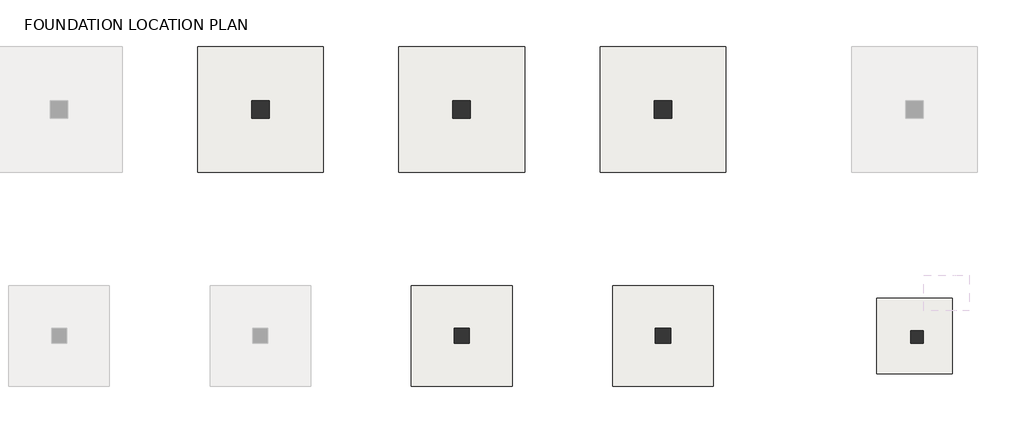
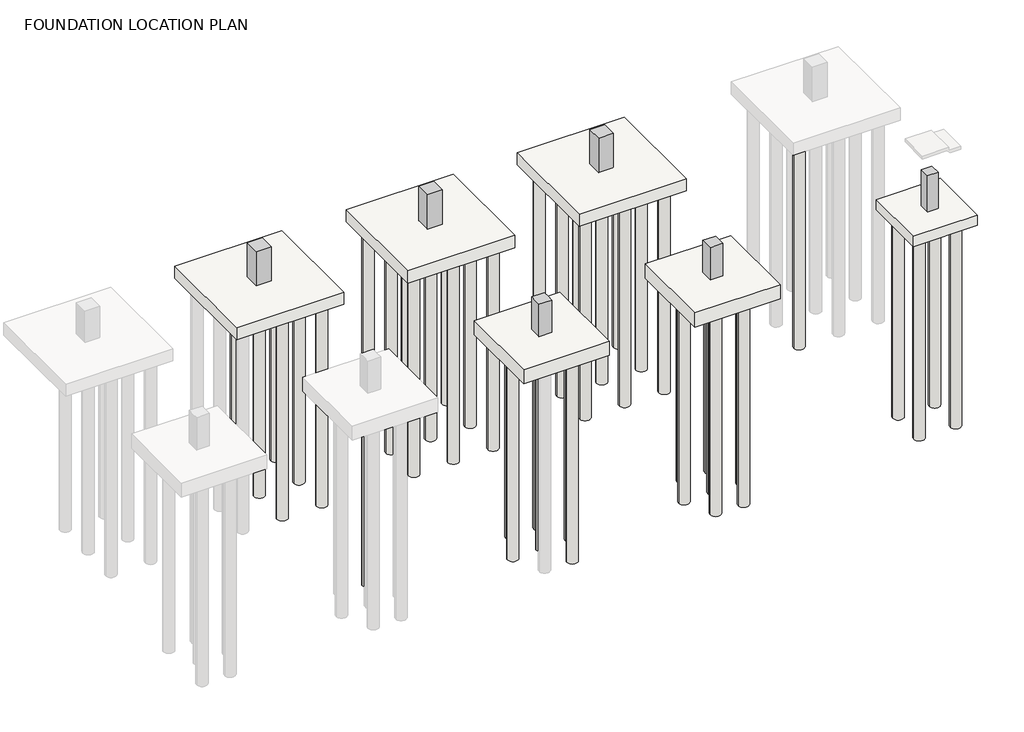
# One storey, part 2 of 3: 49 slabs, 6 columns.
"""IFC4 building model written with IfcOpenShell, lengths in millimetres."""

from ifc_helpers import new_model, si_unit, point, frame, frame_2d, origin, place, context, project, spatial, polyline, circle_curve, trimmed, segment, composite_curve, outline, extrude, faceted_brep, element, save

model = new_model("IFC4")

# Units and contexts
model_context = context("Model", 3, world=origin())
ifc_project = project(units=[si_unit("LENGTHUNIT", "METRE", prefix="MILLI")], contexts=[model_context])

# Site, building, storey
site = spatial("IfcSite", under=ifc_project)
building = spatial("IfcBuilding", under=site)
storey = spatial("IfcBuildingStorey", under=building, Name="FOUNDATION LOCATION PLAN", Elevation=-1699.994759)

# Columns
placement = place(None, origin())
element("IfcColumn", 1, ObjectType="Concrete-Rectangular-Column_R1 : CLS111_RC COLUMN_UG_C1", at=placement, inside=storey, context=model_context, shape_type="Brep", body=[
    faceted_brep([(41850.0, 21199.5208589, -1199.994759), (42350.0, 21199.5208589, -1199.994759), (42350.0, 20699.5208589, -1199.994759), (41850.0, 20699.5208589, -1199.994759), (41850.0, 21199.5208589, 450.005241), (41850.0, 21199.5208589, 600.005241), (42000.0, 21199.5208589, 600.005241), (42350.0, 21199.5208589, 600.005241), (41850.0, 20699.5208589, 600.005241), (41850.0, 20999.5208589, 600.005241), (42350.0, 20699.5208589, 600.005241)], [[[0, 1, 2, 3]], [[1, 0, 4, 5, 6, 7]], [[0, 3, 8, 9, 5, 4]], [[3, 2, 10, 8]], [[2, 1, 7, 10]], [[8, 10, 7, 6, 5, 9]]]),
])
element("IfcColumn", 2, ObjectType="Concrete-Rectangular-Column_R1 : CLS111_RC COLUMN_UG_C3", at=placement, inside=storey, context=model_context, shape_type="Brep", body=[
    faceted_brep([(15650.0, 30349.5208589, -1099.994759), (16350.0, 30349.5208589, -1099.994759), (16350.0, 29649.5208589, -1099.994759), (15650.0, 29649.5208589, -1099.994759), (15650.0, 30349.5208589, 450.005241), (15650.0, 30349.5208589, 600.005241), (16350.0, 30349.5208589, 600.005241), (16350.0, 30349.5208589, 450.005241), (16350.0, 29649.5208589, 600.005241), (16350.0, 29649.5208589, 450.005241), (15650.0, 29649.5208589, 600.005241), (15650.0, 29649.5208589, 450.005241)], [[[0, 1, 2, 3]], [[1, 0, 4, 5, 6, 7]], [[2, 1, 7, 6, 8, 9]], [[3, 2, 9, 8, 10, 11]], [[0, 3, 11, 10, 5, 4]], [[6, 5, 10, 8]]]),
])
element("IfcColumn", 3, ObjectType="Concrete-Rectangular-Column_R1 : CLS111_RC COLUMN_UG_C3", at=placement, inside=storey, context=model_context, shape_type="Brep", body=[
    faceted_brep([(23650.0, 30349.5208589, -1099.994759), (24350.0, 30349.5208589, -1099.994759), (24350.0, 29649.5208589, -1099.994759), (23650.0, 29649.5208589, -1099.994759), (23650.0, 30349.5208589, 450.005241), (23650.0, 30349.5208589, 600.005241), (24350.0, 30349.5208589, 600.005241), (24350.0, 30349.5208589, 450.005241), (24350.0, 29649.5208589, 600.005241), (24350.0, 29649.5208589, 450.005241), (23650.0, 29649.5208589, 600.005241), (23650.0, 29649.5208589, 450.005241)], [[[0, 1, 2, 3]], [[1, 0, 4, 5, 6, 7]], [[2, 1, 7, 6, 8, 9]], [[3, 2, 9, 8, 10, 11]], [[0, 3, 11, 10, 5, 4]], [[6, 5, 10, 8]]]),
])
element("IfcColumn", 4, ObjectType="Concrete-Rectangular-Column_R1 : CLS111_RC COLUMN_UG_C3", at=placement, inside=storey, context=model_context, shape_type="Brep", body=[
    faceted_brep([(31650.0, 30349.5208589, -1099.994759), (32350.0, 30349.5208589, -1099.994759), (32350.0, 29649.5208589, -1099.994759), (31650.0, 29649.5208589, -1099.994759), (31650.0, 30349.5208589, 450.005241), (31650.0, 30349.5208589, 600.005241), (32350.0, 30349.5208589, 600.005241), (32350.0, 30349.5208589, 450.005241), (32350.0, 29649.5208589, 600.005241), (32350.0, 29649.5208589, 450.005241), (31650.0, 29649.5208589, 600.005241), (31650.0, 29649.5208589, 450.005241)], [[[0, 1, 2, 3]], [[1, 0, 4, 5, 6, 7]], [[2, 1, 7, 6, 8, 9]], [[3, 2, 9, 8, 10, 11]], [[0, 3, 11, 10, 5, 4]], [[6, 5, 10, 8]]]),
])
element("IfcColumn", 5, ObjectType="Concrete-Rectangular-Column_R1 : CLS111_RC COLUMN_UG_C2", at=placement, inside=storey, context=model_context, shape_type="Brep", body=[
    faceted_brep([(23700.0, 21299.5208589, -999.994759), (24300.0, 21299.5208589, -999.994759), (24300.0, 20699.5208589, -999.994759), (23700.0, 20699.5208589, -999.994759), (23700.0, 21299.5208589, 450.005241), (23700.0, 21299.5208589, 600.005241), (24300.0, 21299.5208589, 600.005241), (24300.0, 21299.5208589, 450.005241), (24300.0, 20999.5208589, 600.005241), (24300.0, 20699.5208589, 600.005241), (23700.0, 20699.5208589, 600.005241), (23700.0, 20999.5208589, 600.005241)], [[[0, 1, 2, 3]], [[1, 0, 4, 5, 6, 7]], [[2, 1, 7, 6, 8, 9]], [[3, 2, 9, 10]], [[0, 3, 10, 11, 5, 4]], [[6, 5, 11, 10, 9, 8]]]),
])
element("IfcColumn", 6, ObjectType="Concrete-Rectangular-Column_R1 : CLS111_RC COLUMN_UG_C2", at=placement, inside=storey, context=model_context, shape_type="Brep", body=[
    faceted_brep([(31700.0, 21299.5208589, -999.994759), (32300.0, 21299.5208589, -999.994759), (32300.0, 20699.5208589, -999.994759), (31700.0, 20699.5208589, -999.994759), (31700.0, 21299.5208589, 450.005241), (31700.0, 21299.5208589, 600.005241), (32300.0, 21299.5208589, 600.005241), (32300.0, 21299.5208589, 450.005241), (32300.0, 20999.5208589, 600.005241), (32300.0, 20699.5208589, 600.005241), (31700.0, 20699.5208589, 600.005241), (31700.0, 20999.5208589, 600.005241)], [[[0, 1, 2, 3]], [[1, 0, 4, 5, 6, 7]], [[2, 1, 7, 6, 8, 9]], [[3, 2, 9, 10]], [[0, 3, 10, 11, 5, 4]], [[6, 5, 11, 10, 9, 8]]]),
])

# Slabs
element("IfcSlab", 7, ObjectType="Footing-Rectangular_R1 : FTS301_Footing-Rectangular_3000x3000x500_F1", at=placement, inside=storey, context=model_context, shape_type="SweptSolid", body=[
    extrude(outline(polyline([(43500.0, 22499.5208589), (43500.0, 19499.5208589), (40500.0, 19499.5208589), (40500.0, 22499.5208589), (43500.0, 22499.5208589)])), frame((0.0, 0.0, -1699.994759), z_axis=(0.0, 0.0, 1.0), x_axis=(1.0, 0.0, 0.0)), (0.0, 0.0, 1.0), 500.0),
])
element("IfcSlab", 8, ObjectType="Footing-Rectangular_R1 : FTS301_Footing-Rectangular_4000x4000x700_F2", at=placement, inside=storey, context=model_context, shape_type="SweptSolid", body=[
    extrude(outline(polyline([(26000.0, 22999.5208589), (26000.0, 18999.5208589), (22000.0, 18999.5208589), (22000.0, 22999.5208589), (26000.0, 22999.5208589)])), frame((0.0, 0.0, -1699.994759), z_axis=(0.0, 0.0, 1.0), x_axis=(1.0, 0.0, 0.0)), (0.0, 0.0, 1.0), 700.0),
])
element("IfcSlab", 9, ObjectType="Footing-Rectangular_R1 : FTS301_Footing-Rectangular_4000x4000x700_F2", at=placement, inside=storey, context=model_context, shape_type="SweptSolid", body=[
    extrude(outline(polyline([(34000.0, 22999.5208589), (34000.0, 18999.5208589), (30000.0, 18999.5208589), (30000.0, 22999.5208589), (34000.0, 22999.5208589)])), frame((0.0, 0.0, -1699.994759), z_axis=(0.0, 0.0, 1.0), x_axis=(1.0, 0.0, 0.0)), (0.0, 0.0, 1.0), 700.0),
])
element("IfcSlab", 10, ObjectType="Footing-Rectangular_R1 : FTS301_Footing-Rectangular_5000x5000x600_F3", at=placement, inside=storey, context=model_context, shape_type="SweptSolid", body=[
    extrude(outline(polyline([(18500.0, 32499.5208589), (18500.0, 27499.5208589), (13500.0, 27499.5208589), (13500.0, 32499.5208589), (18500.0, 32499.5208589)])), frame((0.0, 0.0, -1699.994759), z_axis=(0.0, 0.0, 1.0), x_axis=(1.0, 0.0, 0.0)), (0.0, 0.0, 1.0), 600.0),
])
element("IfcSlab", 11, ObjectType="Footing-Rectangular_R1 : FTS301_Footing-Rectangular_5000x5000x600_F3", at=placement, inside=storey, context=model_context, shape_type="SweptSolid", body=[
    extrude(outline(polyline([(26500.0, 32499.5208589), (26500.0, 27499.5208589), (21500.0, 27499.5208589), (21500.0, 32499.5208589), (26500.0, 32499.5208589)])), frame((0.0, 0.0, -1699.994759), z_axis=(0.0, 0.0, 1.0), x_axis=(1.0, 0.0, 0.0)), (0.0, 0.0, 1.0), 600.0),
])
element("IfcSlab", 12, ObjectType="Footing-Rectangular_R1 : FTS301_Footing-Rectangular_5000x5000x600_F3", at=placement, inside=storey, context=model_context, shape_type="SweptSolid", body=[
    extrude(outline(polyline([(34500.0, 32499.5208589), (34500.0, 27499.5208589), (29500.0, 27499.5208589), (29500.0, 32499.5208589), (34500.0, 32499.5208589)])), frame((0.0, 0.0, -1699.994759), z_axis=(0.0, 0.0, 1.0), x_axis=(1.0, 0.0, 0.0)), (0.0, 0.0, 1.0), 600.0),
])
element("IfcSlab", 13, ObjectType="HEC_PILE : FTPS102_D500", at=placement, inside=storey, context=model_context, shape_type="SweptSolid", body=[
    extrude(outline(composite_curve([segment(trimmed(circle_curve(frame_2d((41150.0, 21849.5208589)), 250.0), [point((41400.0, 21849.5208589))], [point((40900.0, 21849.5208589))], False, "CARTESIAN"), True, "CONTINUOUS"), segment(trimmed(circle_curve(frame_2d((41150.0, 21849.5208589)), 250.0), [point((40900.0, 21849.5208589))], [point((41400.0, 21849.5208589))], False, "CARTESIAN"), True, "CONTINUOUS")], self_intersect=False)), frame((0.0, 0.0, -11749.994759), z_axis=(0.0, 0.0, 1.0), x_axis=(1.0, 0.0, 0.0)), (0.0, 0.0, 1.0), 10150.0),
])
element("IfcSlab", 14, ObjectType="HEC_PILE : FTPS102_D500", at=placement, inside=storey, context=model_context, shape_type="SweptSolid", body=[
    extrude(outline(composite_curve([segment(trimmed(circle_curve(frame_2d((42850.0, 21849.5208589)), 250.0), [point((42600.0, 21849.5208589))], [point((43100.0, 21849.5208589))], False, "CARTESIAN"), True, "CONTINUOUS"), segment(trimmed(circle_curve(frame_2d((42850.0, 21849.5208589)), 250.0), [point((43100.0, 21849.5208589))], [point((42600.0, 21849.5208589))], False, "CARTESIAN"), True, "CONTINUOUS")], self_intersect=False)), frame((0.0, 0.0, -11749.994759), z_axis=(0.0, 0.0, 1.0), x_axis=(1.0, 0.0, 0.0)), (0.0, 0.0, 1.0), 10150.0),
])
element("IfcSlab", 15, ObjectType="HEC_PILE : FTPS102_D500", at=placement, inside=storey, context=model_context, shape_type="SweptSolid", body=[
    extrude(outline(composite_curve([segment(trimmed(circle_curve(frame_2d((41150.0, 20149.5208589)), 250.0), [point((41400.0, 20149.5208589))], [point((40900.0, 20149.5208589))], False, "CARTESIAN"), True, "CONTINUOUS"), segment(trimmed(circle_curve(frame_2d((41150.0, 20149.5208589)), 250.0), [point((40900.0, 20149.5208589))], [point((41400.0, 20149.5208589))], False, "CARTESIAN"), True, "CONTINUOUS")], self_intersect=False)), frame((0.0, 0.0, -11749.994759), z_axis=(0.0, 0.0, 1.0), x_axis=(1.0, 0.0, 0.0)), (0.0, 0.0, 1.0), 10150.0),
])
element("IfcSlab", 16, ObjectType="HEC_PILE : FTPS102_D500", at=placement, inside=storey, context=model_context, shape_type="SweptSolid", body=[
    extrude(outline(composite_curve([segment(trimmed(circle_curve(frame_2d((42850.0, 20149.5208589)), 250.0), [point((42600.0, 20149.5208589))], [point((43100.0, 20149.5208589))], False, "CARTESIAN"), True, "CONTINUOUS"), segment(trimmed(circle_curve(frame_2d((42850.0, 20149.5208589)), 250.0), [point((43100.0, 20149.5208589))], [point((42600.0, 20149.5208589))], False, "CARTESIAN"), True, "CONTINUOUS")], self_intersect=False)), frame((0.0, 0.0, -11749.994759), z_axis=(0.0, 0.0, 1.0), x_axis=(1.0, 0.0, 0.0)), (0.0, 0.0, 1.0), 10150.0),
])
element("IfcSlab", 17, ObjectType="HEC_PILE : FTPS102_D500", at=placement, inside=storey, context=model_context, shape_type="SweptSolid", body=[
    extrude(outline(composite_curve([segment(trimmed(circle_curve(frame_2d((16650.0, 22349.5208589)), 250.0), [point((16400.0, 22349.5208589))], [point((16900.0, 22349.5208589))], False, "CARTESIAN"), True, "CONTINUOUS"), segment(trimmed(circle_curve(frame_2d((16650.0, 22349.5208589)), 250.0), [point((16900.0, 22349.5208589))], [point((16400.0, 22349.5208589))], False, "CARTESIAN"), True, "CONTINUOUS")], self_intersect=False)), frame((0.0, 0.0, -11749.994759), z_axis=(0.0, 0.0, 1.0), x_axis=(1.0, 0.0, 0.0)), (0.0, 0.0, 1.0), 10150.0),
])
element("IfcSlab", 18, ObjectType="HEC_PILE : FTPS102_D500", at=placement, inside=storey, context=model_context, shape_type="SweptSolid", body=[
    extrude(outline(composite_curve([segment(trimmed(circle_curve(frame_2d((24650.0, 19649.5208589)), 250.0), [point((24400.0, 19649.5208589))], [point((24900.0, 19649.5208589))], False, "CARTESIAN"), True, "CONTINUOUS"), segment(trimmed(circle_curve(frame_2d((24650.0, 19649.5208589)), 250.0), [point((24900.0, 19649.5208589))], [point((24400.0, 19649.5208589))], False, "CARTESIAN"), True, "CONTINUOUS")], self_intersect=False)), frame((0.0, 0.0, -11749.994759), z_axis=(0.0, 0.0, 1.0), x_axis=(1.0, 0.0, 0.0)), (0.0, 0.0, 1.0), 10150.0),
])
element("IfcSlab", 19, ObjectType="HEC_PILE : FTPS102_D500", at=placement, inside=storey, context=model_context, shape_type="SweptSolid", body=[
    extrude(outline(composite_curve([segment(trimmed(circle_curve(frame_2d((22650.0, 20999.5208589)), 250.0), [point((22900.0, 20999.5208589))], [point((22400.0, 20999.5208589))], False, "CARTESIAN"), True, "CONTINUOUS"), segment(trimmed(circle_curve(frame_2d((22650.0, 20999.5208589)), 250.0), [point((22400.0, 20999.5208589))], [point((22900.0, 20999.5208589))], False, "CARTESIAN"), True, "CONTINUOUS")], self_intersect=False)), frame((0.0, 0.0, -11749.994759), z_axis=(0.0, 0.0, 1.0), x_axis=(1.0, 0.0, 0.0)), (0.0, 0.0, 1.0), 10150.0),
])
element("IfcSlab", 20, ObjectType="HEC_PILE : FTPS102_D500", at=placement, inside=storey, context=model_context, shape_type="SweptSolid", body=[
    extrude(outline(composite_curve([segment(trimmed(circle_curve(frame_2d((24000.0, 20999.5208589)), 250.0), [point((24250.0, 20999.5208589))], [point((23750.0, 20999.5208589))], False, "CARTESIAN"), True, "CONTINUOUS"), segment(trimmed(circle_curve(frame_2d((24000.0, 20999.5208589)), 250.0), [point((23750.0, 20999.5208589))], [point((24250.0, 20999.5208589))], False, "CARTESIAN"), True, "CONTINUOUS")], self_intersect=False)), frame((0.0, 0.0, -11749.994759), z_axis=(0.0, 0.0, 1.0), x_axis=(1.0, 0.0, 0.0)), (0.0, 0.0, 1.0), 10150.0),
])
element("IfcSlab", 21, ObjectType="HEC_PILE : FTPS102_D500", at=placement, inside=storey, context=model_context, shape_type="SweptSolid", body=[
    extrude(outline(composite_curve([segment(trimmed(circle_curve(frame_2d((25350.0, 20999.5208589)), 250.0), [point((25100.0, 20999.5208589))], [point((25600.0, 20999.5208589))], False, "CARTESIAN"), True, "CONTINUOUS"), segment(trimmed(circle_curve(frame_2d((25350.0, 20999.5208589)), 250.0), [point((25600.0, 20999.5208589))], [point((25100.0, 20999.5208589))], False, "CARTESIAN"), True, "CONTINUOUS")], self_intersect=False)), frame((0.0, 0.0, -11749.994759), z_axis=(0.0, 0.0, 1.0), x_axis=(1.0, 0.0, 0.0)), (0.0, 0.0, 1.0), 10150.0),
])
element("IfcSlab", 22, ObjectType="HEC_PILE : FTPS102_D500", at=placement, inside=storey, context=model_context, shape_type="SweptSolid", body=[
    extrude(outline(composite_curve([segment(trimmed(circle_curve(frame_2d((23350.0, 22349.5208589)), 250.0), [point((23600.0, 22349.5208589))], [point((23100.0, 22349.5208589))], False, "CARTESIAN"), True, "CONTINUOUS"), segment(trimmed(circle_curve(frame_2d((23350.0, 22349.5208589)), 250.0), [point((23100.0, 22349.5208589))], [point((23600.0, 22349.5208589))], False, "CARTESIAN"), True, "CONTINUOUS")], self_intersect=False)), frame((0.0, 0.0, -11749.994759), z_axis=(0.0, 0.0, 1.0), x_axis=(1.0, 0.0, 0.0)), (0.0, 0.0, 1.0), 10150.0),
])
element("IfcSlab", 23, ObjectType="HEC_PILE : FTPS102_D500", at=placement, inside=storey, context=model_context, shape_type="SweptSolid", body=[
    extrude(outline(composite_curve([segment(trimmed(circle_curve(frame_2d((24650.0, 22349.5208589)), 250.0), [point((24400.0, 22349.5208589))], [point((24900.0, 22349.5208589))], False, "CARTESIAN"), True, "CONTINUOUS"), segment(trimmed(circle_curve(frame_2d((24650.0, 22349.5208589)), 250.0), [point((24900.0, 22349.5208589))], [point((24400.0, 22349.5208589))], False, "CARTESIAN"), True, "CONTINUOUS")], self_intersect=False)), frame((0.0, 0.0, -11749.994759), z_axis=(0.0, 0.0, 1.0), x_axis=(1.0, 0.0, 0.0)), (0.0, 0.0, 1.0), 10150.0),
])
element("IfcSlab", 24, ObjectType="HEC_PILE : FTPS102_D500", at=placement, inside=storey, context=model_context, shape_type="SweptSolid", body=[
    extrude(outline(composite_curve([segment(trimmed(circle_curve(frame_2d((31350.0, 19649.5208589)), 250.0), [point((31600.0, 19649.5208589))], [point((31100.0, 19649.5208589))], False, "CARTESIAN"), True, "CONTINUOUS"), segment(trimmed(circle_curve(frame_2d((31350.0, 19649.5208589)), 250.0), [point((31100.0, 19649.5208589))], [point((31600.0, 19649.5208589))], False, "CARTESIAN"), True, "CONTINUOUS")], self_intersect=False)), frame((0.0, 0.0, -11749.994759), z_axis=(0.0, 0.0, 1.0), x_axis=(1.0, 0.0, 0.0)), (0.0, 0.0, 1.0), 10150.0),
])
element("IfcSlab", 25, ObjectType="HEC_PILE : FTPS102_D500", at=placement, inside=storey, context=model_context, shape_type="SweptSolid", body=[
    extrude(outline(composite_curve([segment(trimmed(circle_curve(frame_2d((32650.0, 19649.5208589)), 250.0), [point((32400.0, 19649.5208589))], [point((32900.0, 19649.5208589))], False, "CARTESIAN"), True, "CONTINUOUS"), segment(trimmed(circle_curve(frame_2d((32650.0, 19649.5208589)), 250.0), [point((32900.0, 19649.5208589))], [point((32400.0, 19649.5208589))], False, "CARTESIAN"), True, "CONTINUOUS")], self_intersect=False)), frame((0.0, 0.0, -11749.994759), z_axis=(0.0, 0.0, 1.0), x_axis=(1.0, 0.0, 0.0)), (0.0, 0.0, 1.0), 10150.0),
])
element("IfcSlab", 26, ObjectType="HEC_PILE : FTPS102_D500", at=placement, inside=storey, context=model_context, shape_type="SweptSolid", body=[
    extrude(outline(composite_curve([segment(trimmed(circle_curve(frame_2d((30650.0, 20999.5208589)), 250.0), [point((30900.0, 20999.5208589))], [point((30400.0, 20999.5208589))], False, "CARTESIAN"), True, "CONTINUOUS"), segment(trimmed(circle_curve(frame_2d((30650.0, 20999.5208589)), 250.0), [point((30400.0, 20999.5208589))], [point((30900.0, 20999.5208589))], False, "CARTESIAN"), True, "CONTINUOUS")], self_intersect=False)), frame((0.0, 0.0, -11749.994759), z_axis=(0.0, 0.0, 1.0), x_axis=(1.0, 0.0, 0.0)), (0.0, 0.0, 1.0), 10150.0),
])
element("IfcSlab", 27, ObjectType="HEC_PILE : FTPS102_D500", at=placement, inside=storey, context=model_context, shape_type="SweptSolid", body=[
    extrude(outline(composite_curve([segment(trimmed(circle_curve(frame_2d((32000.0, 20999.5208589)), 250.0), [point((32250.0, 20999.5208589))], [point((31750.0, 20999.5208589))], False, "CARTESIAN"), True, "CONTINUOUS"), segment(trimmed(circle_curve(frame_2d((32000.0, 20999.5208589)), 250.0), [point((31750.0, 20999.5208589))], [point((32250.0, 20999.5208589))], False, "CARTESIAN"), True, "CONTINUOUS")], self_intersect=False)), frame((0.0, 0.0, -11749.994759), z_axis=(0.0, 0.0, 1.0), x_axis=(1.0, 0.0, 0.0)), (0.0, 0.0, 1.0), 10150.0),
])
element("IfcSlab", 28, ObjectType="HEC_PILE : FTPS102_D500", at=placement, inside=storey, context=model_context, shape_type="SweptSolid", body=[
    extrude(outline(composite_curve([segment(trimmed(circle_curve(frame_2d((33350.0, 20999.5208589)), 250.0), [point((33100.0, 20999.5208589))], [point((33600.0, 20999.5208589))], False, "CARTESIAN"), True, "CONTINUOUS"), segment(trimmed(circle_curve(frame_2d((33350.0, 20999.5208589)), 250.0), [point((33600.0, 20999.5208589))], [point((33100.0, 20999.5208589))], False, "CARTESIAN"), True, "CONTINUOUS")], self_intersect=False)), frame((0.0, 0.0, -11749.994759), z_axis=(0.0, 0.0, 1.0), x_axis=(1.0, 0.0, 0.0)), (0.0, 0.0, 1.0), 10150.0),
])
element("IfcSlab", 29, ObjectType="HEC_PILE : FTPS102_D500", at=placement, inside=storey, context=model_context, shape_type="SweptSolid", body=[
    extrude(outline(composite_curve([segment(trimmed(circle_curve(frame_2d((31350.0, 22349.5208589)), 250.0), [point((31600.0, 22349.5208589))], [point((31100.0, 22349.5208589))], False, "CARTESIAN"), True, "CONTINUOUS"), segment(trimmed(circle_curve(frame_2d((31350.0, 22349.5208589)), 250.0), [point((31100.0, 22349.5208589))], [point((31600.0, 22349.5208589))], False, "CARTESIAN"), True, "CONTINUOUS")], self_intersect=False)), frame((0.0, 0.0, -11749.994759), z_axis=(0.0, 0.0, 1.0), x_axis=(1.0, 0.0, 0.0)), (0.0, 0.0, 1.0), 10150.0),
])
element("IfcSlab", 30, ObjectType="HEC_PILE : FTPS102_D500", at=placement, inside=storey, context=model_context, shape_type="SweptSolid", body=[
    extrude(outline(composite_curve([segment(trimmed(circle_curve(frame_2d((32650.0, 22349.5208589)), 250.0), [point((32400.0, 22349.5208589))], [point((32900.0, 22349.5208589))], False, "CARTESIAN"), True, "CONTINUOUS"), segment(trimmed(circle_curve(frame_2d((32650.0, 22349.5208589)), 250.0), [point((32900.0, 22349.5208589))], [point((32400.0, 22349.5208589))], False, "CARTESIAN"), True, "CONTINUOUS")], self_intersect=False)), frame((0.0, 0.0, -11749.994759), z_axis=(0.0, 0.0, 1.0), x_axis=(1.0, 0.0, 0.0)), (0.0, 0.0, 1.0), 10150.0),
])
element("IfcSlab", 31, ObjectType="HEC_PILE : FTPS102_D500", at=placement, inside=storey, context=model_context, shape_type="SweptSolid", body=[
    extrude(outline(composite_curve([segment(trimmed(circle_curve(frame_2d((17850.0, 29999.5208589)), 250.0), [point((17600.0, 29999.5208589))], [point((18100.0, 29999.5208589))], False, "CARTESIAN"), True, "CONTINUOUS"), segment(trimmed(circle_curve(frame_2d((17850.0, 29999.5208589)), 250.0), [point((18100.0, 29999.5208589))], [point((17600.0, 29999.5208589))], False, "CARTESIAN"), True, "CONTINUOUS")], self_intersect=False)), frame((0.0, 0.0, -11749.994759), z_axis=(0.0, 0.0, 1.0), x_axis=(1.0, 0.0, 0.0)), (0.0, 0.0, 1.0), 10150.0),
])
element("IfcSlab", 32, ObjectType="HEC_PILE : FTPS102_D500", at=placement, inside=storey, context=model_context, shape_type="SweptSolid", body=[
    extrude(outline(composite_curve([segment(trimmed(circle_curve(frame_2d((16000.0, 29999.5208589)), 250.0), [point((15750.0, 29999.5208589))], [point((16250.0, 29999.5208589))], False, "CARTESIAN"), True, "CONTINUOUS"), segment(trimmed(circle_curve(frame_2d((16000.0, 29999.5208589)), 250.0), [point((16250.0, 29999.5208589))], [point((15750.0, 29999.5208589))], False, "CARTESIAN"), True, "CONTINUOUS")], self_intersect=False)), frame((0.0, 0.0, -11749.994759), z_axis=(0.0, 0.0, 1.0), x_axis=(1.0, 0.0, 0.0)), (0.0, 0.0, 1.0), 10150.0),
])
element("IfcSlab", 33, ObjectType="HEC_PILE : FTPS102_D500", at=placement, inside=storey, context=model_context, shape_type="SweptSolid", body=[
    extrude(outline(composite_curve([segment(trimmed(circle_curve(frame_2d((17850.0, 31849.5208589)), 250.0), [point((17600.0, 31849.5208589))], [point((18100.0, 31849.5208589))], False, "CARTESIAN"), True, "CONTINUOUS"), segment(trimmed(circle_curve(frame_2d((17850.0, 31849.5208589)), 250.0), [point((18100.0, 31849.5208589))], [point((17600.0, 31849.5208589))], False, "CARTESIAN"), True, "CONTINUOUS")], self_intersect=False)), frame((0.0, 0.0, -11749.994759), z_axis=(0.0, 0.0, 1.0), x_axis=(1.0, 0.0, 0.0)), (0.0, 0.0, 1.0), 10150.0),
])
element("IfcSlab", 34, ObjectType="HEC_PILE : FTPS102_D500", at=placement, inside=storey, context=model_context, shape_type="SweptSolid", body=[
    extrude(outline(composite_curve([segment(trimmed(circle_curve(frame_2d((16000.0, 31849.5208589)), 250.0), [point((15750.0, 31849.5208589))], [point((16250.0, 31849.5208589))], False, "CARTESIAN"), True, "CONTINUOUS"), segment(trimmed(circle_curve(frame_2d((16000.0, 31849.5208589)), 250.0), [point((16250.0, 31849.5208589))], [point((15750.0, 31849.5208589))], False, "CARTESIAN"), True, "CONTINUOUS")], self_intersect=False)), frame((0.0, 0.0, -11749.994759), z_axis=(0.0, 0.0, 1.0), x_axis=(1.0, 0.0, 0.0)), (0.0, 0.0, 1.0), 10150.0),
])
element("IfcSlab", 35, ObjectType="HEC_PILE : FTPS102_D500", at=placement, inside=storey, context=model_context, shape_type="SweptSolid", body=[
    extrude(outline(composite_curve([segment(trimmed(circle_curve(frame_2d((17850.0, 28149.5208589)), 250.0), [point((17600.0, 28149.5208589))], [point((18100.0, 28149.5208589))], False, "CARTESIAN"), True, "CONTINUOUS"), segment(trimmed(circle_curve(frame_2d((17850.0, 28149.5208589)), 250.0), [point((18100.0, 28149.5208589))], [point((17600.0, 28149.5208589))], False, "CARTESIAN"), True, "CONTINUOUS")], self_intersect=False)), frame((0.0, 0.0, -11749.994759), z_axis=(0.0, 0.0, 1.0), x_axis=(1.0, 0.0, 0.0)), (0.0, 0.0, 1.0), 10150.0),
])
element("IfcSlab", 36, ObjectType="HEC_PILE : FTPS102_D500", at=placement, inside=storey, context=model_context, shape_type="SweptSolid", body=[
    extrude(outline(composite_curve([segment(trimmed(circle_curve(frame_2d((16000.0, 28149.5208589)), 250.0), [point((15750.0, 28149.5208589))], [point((16250.0, 28149.5208589))], False, "CARTESIAN"), True, "CONTINUOUS"), segment(trimmed(circle_curve(frame_2d((16000.0, 28149.5208589)), 250.0), [point((16250.0, 28149.5208589))], [point((15750.0, 28149.5208589))], False, "CARTESIAN"), True, "CONTINUOUS")], self_intersect=False)), frame((0.0, 0.0, -11749.994759), z_axis=(0.0, 0.0, 1.0), x_axis=(1.0, 0.0, 0.0)), (0.0, 0.0, 1.0), 10150.0),
])
element("IfcSlab", 37, ObjectType="HEC_PILE : FTPS102_D500", at=placement, inside=storey, context=model_context, shape_type="SweptSolid", body=[
    extrude(outline(composite_curve([segment(trimmed(circle_curve(frame_2d((22150.0, 29999.5208589)), 250.0), [point((22400.0, 29999.5208589))], [point((21900.0, 29999.5208589))], False, "CARTESIAN"), True, "CONTINUOUS"), segment(trimmed(circle_curve(frame_2d((22150.0, 29999.5208589)), 250.0), [point((21900.0, 29999.5208589))], [point((22400.0, 29999.5208589))], False, "CARTESIAN"), True, "CONTINUOUS")], self_intersect=False)), frame((0.0, 0.0, -11749.994759), z_axis=(0.0, 0.0, 1.0), x_axis=(1.0, 0.0, 0.0)), (0.0, 0.0, 1.0), 10150.0),
])
element("IfcSlab", 38, ObjectType="HEC_PILE : FTPS102_D500", at=placement, inside=storey, context=model_context, shape_type="SweptSolid", body=[
    extrude(outline(composite_curve([segment(trimmed(circle_curve(frame_2d((25850.0, 29999.5208589)), 250.0), [point((25600.0, 29999.5208589))], [point((26100.0, 29999.5208589))], False, "CARTESIAN"), True, "CONTINUOUS"), segment(trimmed(circle_curve(frame_2d((25850.0, 29999.5208589)), 250.0), [point((26100.0, 29999.5208589))], [point((25600.0, 29999.5208589))], False, "CARTESIAN"), True, "CONTINUOUS")], self_intersect=False)), frame((0.0, 0.0, -11749.994759), z_axis=(0.0, 0.0, 1.0), x_axis=(1.0, 0.0, 0.0)), (0.0, 0.0, 1.0), 10150.0),
])
element("IfcSlab", 39, ObjectType="HEC_PILE : FTPS102_D500", at=placement, inside=storey, context=model_context, shape_type="SweptSolid", body=[
    extrude(outline(composite_curve([segment(trimmed(circle_curve(frame_2d((24000.0, 29999.5208589)), 250.0), [point((23750.0, 29999.5208589))], [point((24250.0, 29999.5208589))], False, "CARTESIAN"), True, "CONTINUOUS"), segment(trimmed(circle_curve(frame_2d((24000.0, 29999.5208589)), 250.0), [point((24250.0, 29999.5208589))], [point((23750.0, 29999.5208589))], False, "CARTESIAN"), True, "CONTINUOUS")], self_intersect=False)), frame((0.0, 0.0, -11749.994759), z_axis=(0.0, 0.0, 1.0), x_axis=(1.0, 0.0, 0.0)), (0.0, 0.0, 1.0), 10150.0),
])
element("IfcSlab", 40, ObjectType="HEC_PILE : FTPS102_D500", at=placement, inside=storey, context=model_context, shape_type="SweptSolid", body=[
    extrude(outline(composite_curve([segment(trimmed(circle_curve(frame_2d((22150.0, 31849.5208589)), 250.0), [point((22400.0, 31849.5208589))], [point((21900.0, 31849.5208589))], False, "CARTESIAN"), True, "CONTINUOUS"), segment(trimmed(circle_curve(frame_2d((22150.0, 31849.5208589)), 250.0), [point((21900.0, 31849.5208589))], [point((22400.0, 31849.5208589))], False, "CARTESIAN"), True, "CONTINUOUS")], self_intersect=False)), frame((0.0, 0.0, -11749.994759), z_axis=(0.0, 0.0, 1.0), x_axis=(1.0, 0.0, 0.0)), (0.0, 0.0, 1.0), 10150.0),
])
element("IfcSlab", 41, ObjectType="HEC_PILE : FTPS102_D500", at=placement, inside=storey, context=model_context, shape_type="SweptSolid", body=[
    extrude(outline(composite_curve([segment(trimmed(circle_curve(frame_2d((25850.0, 31849.5208589)), 250.0), [point((25600.0, 31849.5208589))], [point((26100.0, 31849.5208589))], False, "CARTESIAN"), True, "CONTINUOUS"), segment(trimmed(circle_curve(frame_2d((25850.0, 31849.5208589)), 250.0), [point((26100.0, 31849.5208589))], [point((25600.0, 31849.5208589))], False, "CARTESIAN"), True, "CONTINUOUS")], self_intersect=False)), frame((0.0, 0.0, -11749.994759), z_axis=(0.0, 0.0, 1.0), x_axis=(1.0, 0.0, 0.0)), (0.0, 0.0, 1.0), 10150.0),
])
element("IfcSlab", 42, ObjectType="HEC_PILE : FTPS102_D500", at=placement, inside=storey, context=model_context, shape_type="SweptSolid", body=[
    extrude(outline(composite_curve([segment(trimmed(circle_curve(frame_2d((24000.0, 31849.5208589)), 250.0), [point((23750.0, 31849.5208589))], [point((24250.0, 31849.5208589))], False, "CARTESIAN"), True, "CONTINUOUS"), segment(trimmed(circle_curve(frame_2d((24000.0, 31849.5208589)), 250.0), [point((24250.0, 31849.5208589))], [point((23750.0, 31849.5208589))], False, "CARTESIAN"), True, "CONTINUOUS")], self_intersect=False)), frame((0.0, 0.0, -11749.994759), z_axis=(0.0, 0.0, 1.0), x_axis=(1.0, 0.0, 0.0)), (0.0, 0.0, 1.0), 10150.0),
])
element("IfcSlab", 43, ObjectType="HEC_PILE : FTPS102_D500", at=placement, inside=storey, context=model_context, shape_type="SweptSolid", body=[
    extrude(outline(composite_curve([segment(trimmed(circle_curve(frame_2d((22150.0, 28149.5208589)), 250.0), [point((22400.0, 28149.5208589))], [point((21900.0, 28149.5208589))], False, "CARTESIAN"), True, "CONTINUOUS"), segment(trimmed(circle_curve(frame_2d((22150.0, 28149.5208589)), 250.0), [point((21900.0, 28149.5208589))], [point((22400.0, 28149.5208589))], False, "CARTESIAN"), True, "CONTINUOUS")], self_intersect=False)), frame((0.0, 0.0, -11749.994759), z_axis=(0.0, 0.0, 1.0), x_axis=(1.0, 0.0, 0.0)), (0.0, 0.0, 1.0), 10150.0),
])
element("IfcSlab", 44, ObjectType="HEC_PILE : FTPS102_D500", at=placement, inside=storey, context=model_context, shape_type="SweptSolid", body=[
    extrude(outline(composite_curve([segment(trimmed(circle_curve(frame_2d((25850.0, 28149.5208589)), 250.0), [point((25600.0, 28149.5208589))], [point((26100.0, 28149.5208589))], False, "CARTESIAN"), True, "CONTINUOUS"), segment(trimmed(circle_curve(frame_2d((25850.0, 28149.5208589)), 250.0), [point((26100.0, 28149.5208589))], [point((25600.0, 28149.5208589))], False, "CARTESIAN"), True, "CONTINUOUS")], self_intersect=False)), frame((0.0, 0.0, -11749.994759), z_axis=(0.0, 0.0, 1.0), x_axis=(1.0, 0.0, 0.0)), (0.0, 0.0, 1.0), 10150.0),
])
element("IfcSlab", 45, ObjectType="HEC_PILE : FTPS102_D500", at=placement, inside=storey, context=model_context, shape_type="SweptSolid", body=[
    extrude(outline(composite_curve([segment(trimmed(circle_curve(frame_2d((24000.0, 28149.5208589)), 250.0), [point((23750.0, 28149.5208589))], [point((24250.0, 28149.5208589))], False, "CARTESIAN"), True, "CONTINUOUS"), segment(trimmed(circle_curve(frame_2d((24000.0, 28149.5208589)), 250.0), [point((24250.0, 28149.5208589))], [point((23750.0, 28149.5208589))], False, "CARTESIAN"), True, "CONTINUOUS")], self_intersect=False)), frame((0.0, 0.0, -11749.994759), z_axis=(0.0, 0.0, 1.0), x_axis=(1.0, 0.0, 0.0)), (0.0, 0.0, 1.0), 10150.0),
])
element("IfcSlab", 46, ObjectType="HEC_PILE : FTPS102_D500", at=placement, inside=storey, context=model_context, shape_type="SweptSolid", body=[
    extrude(outline(composite_curve([segment(trimmed(circle_curve(frame_2d((30150.0, 29999.5208589)), 250.0), [point((30400.0, 29999.5208589))], [point((29900.0, 29999.5208589))], False, "CARTESIAN"), True, "CONTINUOUS"), segment(trimmed(circle_curve(frame_2d((30150.0, 29999.5208589)), 250.0), [point((29900.0, 29999.5208589))], [point((30400.0, 29999.5208589))], False, "CARTESIAN"), True, "CONTINUOUS")], self_intersect=False)), frame((0.0, 0.0, -11749.994759), z_axis=(0.0, 0.0, 1.0), x_axis=(1.0, 0.0, 0.0)), (0.0, 0.0, 1.0), 10150.0),
])
element("IfcSlab", 47, ObjectType="HEC_PILE : FTPS102_D500", at=placement, inside=storey, context=model_context, shape_type="SweptSolid", body=[
    extrude(outline(composite_curve([segment(trimmed(circle_curve(frame_2d((33850.0, 29999.5208589)), 250.0), [point((33600.0, 29999.5208589))], [point((34100.0, 29999.5208589))], False, "CARTESIAN"), True, "CONTINUOUS"), segment(trimmed(circle_curve(frame_2d((33850.0, 29999.5208589)), 250.0), [point((34100.0, 29999.5208589))], [point((33600.0, 29999.5208589))], False, "CARTESIAN"), True, "CONTINUOUS")], self_intersect=False)), frame((0.0, 0.0, -11749.994759), z_axis=(0.0, 0.0, 1.0), x_axis=(1.0, 0.0, 0.0)), (0.0, 0.0, 1.0), 10150.0),
])
element("IfcSlab", 48, ObjectType="HEC_PILE : FTPS102_D500", at=placement, inside=storey, context=model_context, shape_type="SweptSolid", body=[
    extrude(outline(composite_curve([segment(trimmed(circle_curve(frame_2d((32000.0, 29999.5208589)), 250.0), [point((31750.0, 29999.5208589))], [point((32250.0, 29999.5208589))], False, "CARTESIAN"), True, "CONTINUOUS"), segment(trimmed(circle_curve(frame_2d((32000.0, 29999.5208589)), 250.0), [point((32250.0, 29999.5208589))], [point((31750.0, 29999.5208589))], False, "CARTESIAN"), True, "CONTINUOUS")], self_intersect=False)), frame((0.0, 0.0, -11749.994759), z_axis=(0.0, 0.0, 1.0), x_axis=(1.0, 0.0, 0.0)), (0.0, 0.0, 1.0), 10150.0),
])
element("IfcSlab", 49, ObjectType="HEC_PILE : FTPS102_D500", at=placement, inside=storey, context=model_context, shape_type="SweptSolid", body=[
    extrude(outline(composite_curve([segment(trimmed(circle_curve(frame_2d((30150.0, 31849.5208589)), 250.0), [point((30400.0, 31849.5208589))], [point((29900.0, 31849.5208589))], False, "CARTESIAN"), True, "CONTINUOUS"), segment(trimmed(circle_curve(frame_2d((30150.0, 31849.5208589)), 250.0), [point((29900.0, 31849.5208589))], [point((30400.0, 31849.5208589))], False, "CARTESIAN"), True, "CONTINUOUS")], self_intersect=False)), frame((0.0, 0.0, -11749.994759), z_axis=(0.0, 0.0, 1.0), x_axis=(1.0, 0.0, 0.0)), (0.0, 0.0, 1.0), 10150.0),
])
element("IfcSlab", 50, ObjectType="HEC_PILE : FTPS102_D500", at=placement, inside=storey, context=model_context, shape_type="SweptSolid", body=[
    extrude(outline(composite_curve([segment(trimmed(circle_curve(frame_2d((33850.0, 31849.5208589)), 250.0), [point((33600.0, 31849.5208589))], [point((34100.0, 31849.5208589))], False, "CARTESIAN"), True, "CONTINUOUS"), segment(trimmed(circle_curve(frame_2d((33850.0, 31849.5208589)), 250.0), [point((34100.0, 31849.5208589))], [point((33600.0, 31849.5208589))], False, "CARTESIAN"), True, "CONTINUOUS")], self_intersect=False)), frame((0.0, 0.0, -11749.994759), z_axis=(0.0, 0.0, 1.0), x_axis=(1.0, 0.0, 0.0)), (0.0, 0.0, 1.0), 10150.0),
])
element("IfcSlab", 51, ObjectType="HEC_PILE : FTPS102_D500", at=placement, inside=storey, context=model_context, shape_type="SweptSolid", body=[
    extrude(outline(composite_curve([segment(trimmed(circle_curve(frame_2d((32000.0, 31849.5208589)), 250.0), [point((31750.0, 31849.5208589))], [point((32250.0, 31849.5208589))], False, "CARTESIAN"), True, "CONTINUOUS"), segment(trimmed(circle_curve(frame_2d((32000.0, 31849.5208589)), 250.0), [point((32250.0, 31849.5208589))], [point((31750.0, 31849.5208589))], False, "CARTESIAN"), True, "CONTINUOUS")], self_intersect=False)), frame((0.0, 0.0, -11749.994759), z_axis=(0.0, 0.0, 1.0), x_axis=(1.0, 0.0, 0.0)), (0.0, 0.0, 1.0), 10150.0),
])
element("IfcSlab", 52, ObjectType="HEC_PILE : FTPS102_D500", at=placement, inside=storey, context=model_context, shape_type="SweptSolid", body=[
    extrude(outline(composite_curve([segment(trimmed(circle_curve(frame_2d((30150.0, 28149.5208589)), 250.0), [point((30400.0, 28149.5208589))], [point((29900.0, 28149.5208589))], False, "CARTESIAN"), True, "CONTINUOUS"), segment(trimmed(circle_curve(frame_2d((30150.0, 28149.5208589)), 250.0), [point((29900.0, 28149.5208589))], [point((30400.0, 28149.5208589))], False, "CARTESIAN"), True, "CONTINUOUS")], self_intersect=False)), frame((0.0, 0.0, -11749.994759), z_axis=(0.0, 0.0, 1.0), x_axis=(1.0, 0.0, 0.0)), (0.0, 0.0, 1.0), 10150.0),
])
element("IfcSlab", 53, ObjectType="HEC_PILE : FTPS102_D500", at=placement, inside=storey, context=model_context, shape_type="SweptSolid", body=[
    extrude(outline(composite_curve([segment(trimmed(circle_curve(frame_2d((33850.0, 28149.5208589)), 250.0), [point((33600.0, 28149.5208589))], [point((34100.0, 28149.5208589))], False, "CARTESIAN"), True, "CONTINUOUS"), segment(trimmed(circle_curve(frame_2d((33850.0, 28149.5208589)), 250.0), [point((34100.0, 28149.5208589))], [point((33600.0, 28149.5208589))], False, "CARTESIAN"), True, "CONTINUOUS")], self_intersect=False)), frame((0.0, 0.0, -11749.994759), z_axis=(0.0, 0.0, 1.0), x_axis=(1.0, 0.0, 0.0)), (0.0, 0.0, 1.0), 10150.0),
])
element("IfcSlab", 54, ObjectType="HEC_PILE : FTPS102_D500", at=placement, inside=storey, context=model_context, shape_type="SweptSolid", body=[
    extrude(outline(composite_curve([segment(trimmed(circle_curve(frame_2d((32000.0, 28149.5208589)), 250.0), [point((31750.0, 28149.5208589))], [point((32250.0, 28149.5208589))], False, "CARTESIAN"), True, "CONTINUOUS"), segment(trimmed(circle_curve(frame_2d((32000.0, 28149.5208589)), 250.0), [point((32250.0, 28149.5208589))], [point((31750.0, 28149.5208589))], False, "CARTESIAN"), True, "CONTINUOUS")], self_intersect=False)), frame((0.0, 0.0, -11749.994759), z_axis=(0.0, 0.0, 1.0), x_axis=(1.0, 0.0, 0.0)), (0.0, 0.0, 1.0), 10150.0),
])
element("IfcSlab", 55, ObjectType="HEC_PILE : FTPS102_D500", at=placement, inside=storey, context=model_context, shape_type="SweptSolid", body=[
    extrude(outline(composite_curve([segment(trimmed(circle_curve(frame_2d((40150.0, 28149.5208589)), 250.0), [point((40400.0, 28149.5208589))], [point((39900.0, 28149.5208589))], False, "CARTESIAN"), True, "CONTINUOUS"), segment(trimmed(circle_curve(frame_2d((40150.0, 28149.5208589)), 250.0), [point((39900.0, 28149.5208589))], [point((40400.0, 28149.5208589))], False, "CARTESIAN"), True, "CONTINUOUS")], self_intersect=False)), frame((0.0, 0.0, -11749.994759), z_axis=(0.0, 0.0, 1.0), x_axis=(1.0, 0.0, 0.0)), (0.0, 0.0, 1.0), 10150.0),
])

save(model, "model.ifc")

# Revit data of these elements
# Type "Concrete-Rectangular-Column_R1 : CLS111_RC COLUMN_UG_C1"
#   Description = "AG RC 기둥"
#   Width = 500 mm
#   Length = 500 mm
#   hec_material3 [instance default] = none
#   hec_material2 [instance default] = A03AE056-00001_Bitumen/Bituminous/Asphalt Coating
#   hec_material1 [instance default] = A03AC035-00001_Form Work (3 times in use)_Flat
#   Structural Material [instance default] = A03AC032-00007_Structural Concrete_Type1_25MPa-30Mpa
# Type "Concrete-Rectangular-Column_R1 : CLS111_RC COLUMN_UG_C3"
#   Description = "AG RC 기둥"
#   Width = 700 mm
#   Length = 700 mm
#   hec_material3 [instance default] = none
#   hec_material2 [instance default] = A03AE056-00001_Bitumen/Bituminous/Asphalt Coating
#   hec_material1 [instance default] = A03AC035-00001_Form Work (3 times in use)_Flat
#   Structural Material [instance default] = A03AC032-00007_Structural Concrete_Type1_25MPa-30Mpa
# Type "Concrete-Rectangular-Column_R1 : CLS111_RC COLUMN_UG_C2"
#   Description = "AG RC 기둥"
#   Width = 600 mm
#   Length = 600 mm
#   hec_material3 [instance default] = none
#   hec_material2 [instance default] = A03AE056-00001_Bitumen/Bituminous/Asphalt Coating
#   hec_material1 [instance default] = A03AC035-00001_Form Work (3 times in use)_Flat
#   Structural Material [instance default] = A03AC032-00007_Structural Concrete_Type1_25MPa-30Mpa
# Type "Footing-Rectangular_R1 : FTS301_Footing-Rectangular_3000x3000x500_F1"
#   Type Mark = "F1"
#   Top bar = "D25@300"
#   Description = "UG Shallow Foundation"
#   Bottom bar = "D20@300"
#   Width = 3000 mm
#   Length = 3000 mm
#   Foundation Thickness = 500 mm
#   Structural Material [instance default] = A03AC032-00007_Structural Concrete_Type1_25MPa-30Mpa
#   Assembly Code = ""
# Type "Footing-Rectangular_R1 : FTS301_Footing-Rectangular_4000x4000x700_F2"
#   Type Mark = "F2"
#   Top bar = "D25@300"
#   Description = "UG Shallow Foundation"
#   Bottom bar = "D20@300"
#   Width = 4000 mm
#   Length = 4000 mm
#   Foundation Thickness = 700 mm
#   Structural Material [instance default] = A03AC032-00007_Structural Concrete_Type1_25MPa-30Mpa
#   Assembly Code = ""
# Type "Footing-Rectangular_R1 : FTS301_Footing-Rectangular_5000x5000x600_F3"
#   Type Mark = "F3"
#   Top bar = "D25@300"
#   Description = "UG Shallow Foundation"
#   Bottom bar = "D20@300"
#   Width = 5000 mm
#   Length = 5000 mm
#   Foundation Thickness = 600 mm
#   Structural Material [instance default] = A03AC032-00007_Structural Concrete_Type1_25MPa-30Mpa
#   Assembly Code = ""
# Type "HEC_PILE : FTPS102_D500"
#   Assembly Code = "A1020130"
#   반지름 = 250 mm
#   최소 내포 = 150 mm
#   Diameter = 500 mm
#   Depth = 10000 mm
#   구조 재료 = A02AA014-00001_Piling Work_Reinforced Concrete Pile(Round Type)_Direct Driving
# Element 1 (IfcColumn, "Concrete-Rectangular-Column_R1 : CLS111_RC COLUMN_UG_C1")
#   Mark = "C1"
#   Structural Material = A03AC032-00007_Structural Concrete_Type1_25MPa-30Mpa
#   hec_material3 = none
#   hec_material2 = A03AE056-00001_Bitumen/Bituminous/Asphalt Coating
#   hec_material1 = A03AC035-00001_Form Work (3 times in use)_Flat
#   Phase Created = New Construction
#   Materials on its faces: "A03AC032-00007_Structural Concrete_Type1_25MPa-30Mpa"
# Elements 2, 3, 4 (IfcColumn, "Concrete-Rectangular-Column_R1 : CLS111_RC COLUMN_UG_C3")
#   Mark = "C3"
#   Structural Material = A03AC032-00007_Structural Concrete_Type1_25MPa-30Mpa
#   hec_material3 = none
#   hec_material2 = A03AE056-00001_Bitumen/Bituminous/Asphalt Coating
#   hec_material1 = A03AC035-00001_Form Work (3 times in use)_Flat
#   Phase Created = New Construction
#   Materials on its faces: "A03AC032-00007_Structural Concrete_Type1_25MPa-30Mpa"
# Elements 5, 6 (IfcColumn, "Concrete-Rectangular-Column_R1 : CLS111_RC COLUMN_UG_C2")
#   Mark = "C2"
#   Structural Material = A03AC032-00007_Structural Concrete_Type1_25MPa-30Mpa
#   hec_material3 = none
#   hec_material2 = A03AE056-00001_Bitumen/Bituminous/Asphalt Coating
#   hec_material1 = A03AC035-00001_Form Work (3 times in use)_Flat
#   Phase Created = New Construction
#   Materials on its faces: "A03AC032-00007_Structural Concrete_Type1_25MPa-30Mpa"
# Element 7 (IfcSlab, "Footing-Rectangular_R1 : FTS301_Footing-Rectangular_3000x3000x500_F1")
#   Comments = ""
#   Structural Material = A03AC032-00007_Structural Concrete_Type1_25MPa-30Mpa
#   Phase Created = New Construction
#   Materials on its faces: "A03AC032-00007_Structural Concrete_Type1_25MPa-30Mpa"
# Elements 8, 9 (IfcSlab, "Footing-Rectangular_R1 : FTS301_Footing-Rectangular_4000x4000x700_F2")
#   Comments = ""
#   Structural Material = A03AC032-00007_Structural Concrete_Type1_25MPa-30Mpa
#   Phase Created = New Construction
#   Materials on its faces: "A03AC032-00007_Structural Concrete_Type1_25MPa-30Mpa"
# Elements 10, 11, 12 (IfcSlab, "Footing-Rectangular_R1 : FTS301_Footing-Rectangular_5000x5000x600_F3")
#   Comments = ""
#   Structural Material = A03AC032-00007_Structural Concrete_Type1_25MPa-30Mpa
#   Phase Created = New Construction
#   Materials on its faces: "A03AC032-00007_Structural Concrete_Type1_25MPa-30Mpa"
# Elements 13, 14, 15, 16, 17, 18, 19, 20, 21, 22, 23, 24, 25, 26, 27, 28, 29, 30, 31, 32, 33, 34, 35, 36, 37, 38, 39, 40, 41, 42, 43, 44, 45, 46, 47, 48, 49, 50, 51, 52, 53, 54, 55 (IfcSlab, "HEC_PILE : FTPS102_D500")
#   F01) Building Name = "STEAM TURBINE BLDG"
#   Phase Created = New Construction
#   Materials on its faces: "A02AA014-00001_Piling Work_Reinforced Concrete Pile(Round Type)_Direct Driving"
# Materials
#   "A03AE056-00001_Bitumen/Bituminous/Asphalt Coating": class "Generic", colour RGB 17 17 17, transparency 0, Description = "Damp-proofing", W00) Work Master Code = "A03AE056-00001", W01) Work Master_Lv1 = "Concrete Work", W02) Work Master_Lv2 = "Concrete Protective Coating (U/G)", W03) Work Master_Spec.1 = "Bitumen/Bituminous/Asphalt Coating", Cost = 0
#   "A03AC035-00001_Form Work (3 times in use)_Flat": class "Wood", colour RGB 149 120 74, transparency 0, Description = "Plywood", W00) Work Master Code = "A03AC035-00001", W01) Work Master_Lv1 = "Concrete Work", W02) Work Master_Lv2 = "Substructure Work", W03) Work Master_Spec.1 = "Form Work (3 times in use)", W04) Work Master_Spec.2 = "Flat Form", W05) Work Master_Spec.3 = "Dressed Lumber, Plywood or Steel Form(Wood Planks are not Allowed) incl. Chamfer", Cost = 0
#   "A03AC032-00007_Structural Concrete_Type1_25MPa-30Mpa": class "Concrete", colour RGB 176 176 176, transparency 0, Keynote = "09910.A1", Description = "Reinf. Conc.", W00) Work Master Code = "A03AC032-00007", W01) Work Master_Lv1 = "Concrete Work", W02) Work Master_Lv2 = "Substructure Work", W03) Work Master_Spec.1 = "Structural Concrete", W04) Work Master_Spec.2 = "Cement Type-1", W05) Work Master_Spec.3 = "25MPa < F'c (Cylinder Strength) ≤ 30MPa", Cost = 0
#   "A02AA014-00001_Piling Work_Reinforced Concrete Pile(Round Type)_Direct Driving": class "Concrete", colour RGB 176 176 176, transparency 0, Keynote = "09910.A1", Description = "Reinf. Conc.", Cost = 0
